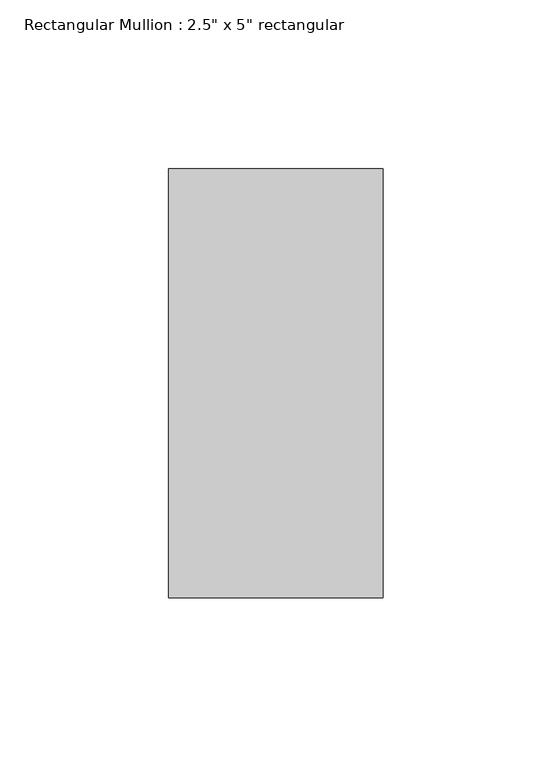
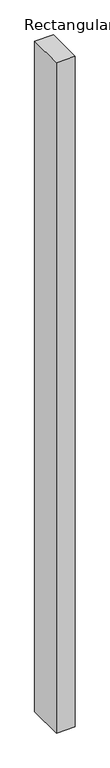
"""IFC4 building model written with IfcOpenShell, lengths in millimetres: member geometry."""

from ifc_helpers import new_model, si_unit, frame, origin, place, context, project, spatial, polyline, outline, extrude, source, transform, mapped, element, save


def member_387659cc(model_context):
    return source(origin(), model_context, "Body", "SweptSolid", [
        extrude(outline(polyline([(0.0, 63.5), (0.0, -63.5), (-63.5, -63.5), (-63.5, 63.5), (0.0, 63.5)])), frame((0.0, 0.0, -2406.65), z_axis=(0.0, 0.0, 1.0), x_axis=(1.0, 0.0, 0.0)), (0.0, 0.0, 1.0), 2406.65),
    ])


if __name__ == "__main__":
    model = new_model("IFC4")
    model_context = context("Model", 3, world=origin())
    ifc_project = project(units=[si_unit("LENGTHUNIT", "METRE", prefix="MILLI")], contexts=[model_context])
    site = spatial("IfcSite", under=ifc_project)
    building = spatial("IfcBuilding", under=site)
    placement = place(None, origin())
    member_shape = member_387659cc(model_context)
    element("IfcMember", 1, ObjectType="Rectangular Mullion : 2.5\" x 5\" rectangular", at=placement, inside=building, context=model_context, shape_type="MappedRepresentation", body=[
        mapped(member_shape, transform((0.0, 0.0, 0.0), x_axis=(1.0, 0.0, 0.0), y_axis=(0.0, 1.0, 0.0), z_axis=(0.0, 0.0, 1.0))),
    ])
    save(model, "model.ifc")

# Revit data of these elements
# Type "Rectangular Mullion : 2.5\" x 5\" rectangular"
#   built-in parameter 1007304 = 0.416667 (stored number, unit not read)
#   built-in parameter 1007301 = 0.104167 (stored number, unit not read)
#   built-in parameter 1007300 = 0.104167 (stored number, unit not read)
# Element 1 (IfcMember, "Rectangular Mullion : 2.5\" x 5\" rectangular")
#   Materials on its faces: "Aluminum"
# Materials
#   "Aluminum": class "Metal", colour RGB 247 247 247, transparency 0, Description = "Aluminum 6061", Cost = 0
